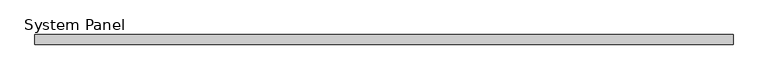
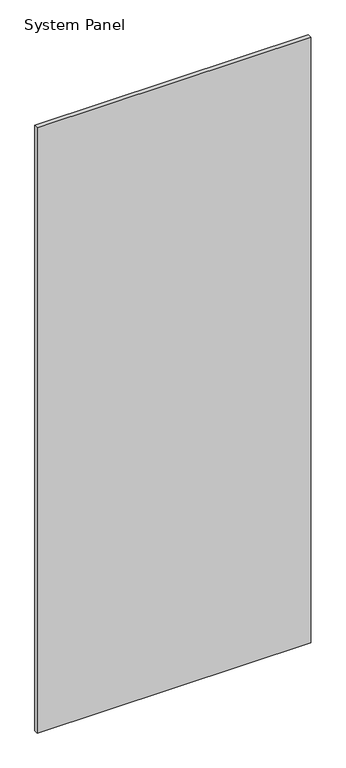
"""IFC4 building model written with IfcOpenShell, lengths in millimetres: plate geometry, System Panel : WWm-Glass-20mm-10mmOffset."""

from ifc_helpers import new_model, si_unit, origin, origin_with_axes, place, context, project, spatial, polyline, outline, extrude, source, transform, mapped, element, save


def system_panel_14e15d3c(model_context):
    return source(origin(), model_context, "Body", "SweptSolid", [
        extrude(outline(polyline([(705.153103, 0.0), (-705.153103, 0.0), (-705.153103, 20.0), (705.153103, 20.0), (705.153103, 0.0)])), origin_with_axes(), (0.0, 0.0, 1.0), 3300.0),
    ])


if __name__ == "__main__":
    model = new_model("IFC4")
    model_context = context("Model", 3, world=origin())
    ifc_project = project(units=[si_unit("LENGTHUNIT", "METRE", prefix="MILLI")], contexts=[model_context])
    site = spatial("IfcSite", under=ifc_project)
    building = spatial("IfcBuilding", under=site)
    placement = place(None, origin())
    system_panel_shape = system_panel_14e15d3c(model_context)
    element("IfcPlate", 1, ObjectType="System Panel : WWm-Glass-20mm-10mmOffset", at=placement, inside=building, context=model_context, shape_type="MappedRepresentation", body=[
        mapped(system_panel_shape, transform((0.0, 0.0, 0.0), x_axis=(1.0, 0.0, 0.0), y_axis=(0.0, 1.0, 0.0), z_axis=(0.0, 0.0, 1.0))),
    ])
    save(model, "model.ifc")

# Revit data of these elements
# Type "System Panel : WWm-Glass-20mm-10mmOffset"
#   Finish = ""
# Element 1 (IfcPlate, "System Panel : WWm-Glass-20mm-10mmOffset")
#   Materials on its faces: "WW-EC-GL-Storefront"
# Materials
#   "WW-EC-GL-Storefront": class "Glass", colour RGB 236 240 239, transparency 0.85, Description = "Storefront Glass", Cost = 0
